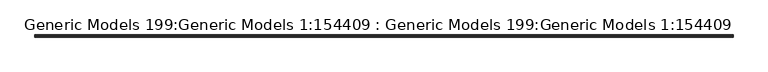
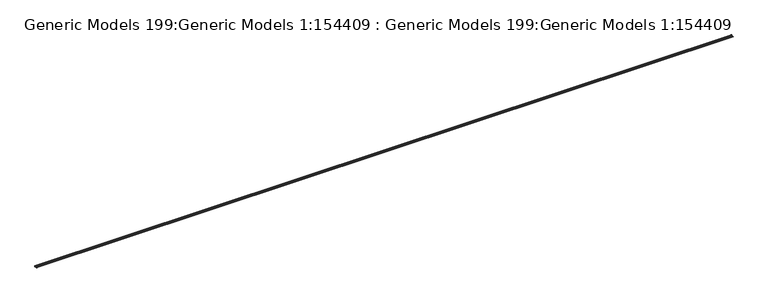
"""IFC4 building model written with IfcOpenShell, lengths in millimetres: proxy geometry, Generic Models 199:Generic Models 1:154409 : Generic Models 199:Generic Models 1:154409."""

from ifc_helpers import new_model, si_unit, frame, origin, place, context, project, spatial, polyline, outline, extrude, source, transform, mapped, element, save


def generic_models_199_generic_models_1_154409_generic_models_aefc242c(model_context):
    return source(origin(), model_context, "Body", "SweptSolid", [
        extrude(outline(polyline([(12159.4075942, 3046.095), (12179.0925942, 3046.095), (12179.0925942, 3048.3048), (12178.2337533, 3048.3048), (12178.2337533, 3068.6193787), (12179.5037533, 3068.6193787), (12179.5037533, 3049.5748), (12180.3625942, 3049.5748), (12180.3625942, 3044.825), (12158.1375942, 3044.825), (12158.1375942, 3056.255), (12145.4375942, 3056.255), (12145.4375942, 3044.825), (12121.7244102, 3044.825), (12121.7244102, 3046.095), (12144.1675942, 3046.095), (12144.1675942, 3057.525), (12159.4075942, 3057.525), (12159.4075942, 3046.095)])), frame((-10588.6040248, 0.0, 0.0), z_axis=(1.0, 0.0, 0.0), x_axis=(0.0, 1.0, 0.0)), (0.0, 0.0, 1.0), 19050.0),
    ])


if __name__ == "__main__":
    model = new_model("IFC4")
    model_context = context("Model", 3, world=origin())
    ifc_project = project(units=[si_unit("LENGTHUNIT", "METRE", prefix="MILLI")], contexts=[model_context])
    site = spatial("IfcSite", under=ifc_project)
    building = spatial("IfcBuilding", under=site)
    placement = place(None, origin())
    generic_models_199_generic_models_1_154409_generic_models_shape = generic_models_199_generic_models_1_154409_generic_models_aefc242c(model_context)
    element("IfcBuildingElementProxy", 1, Name="Generic Models 199:Generic Models 1:154409 : Generic Models 199:Generic Models 1:154409", ObjectType="Generic Models 199:Generic Models 1:154409 : Generic Models 199:Generic Models 1:154409", at=placement, inside=building, context=model_context, shape_type="MappedRepresentation", body=[
        mapped(generic_models_199_generic_models_1_154409_generic_models_shape, transform((0.0, 0.0, 0.0), x_axis=(1.0, 0.0, 0.0), y_axis=(0.0, 1.0, 0.0), z_axis=(0.0, 0.0, 1.0))),
    ])
    save(model, "model.ifc")

# Revit data of these elements
# Type "Generic Models 199:Generic Models 1:154409 : Generic Models 199:Generic Models 1:154409"
#   NameOverride = "Generic Models 199:Generic Models 1:154409"
#   ObjectTypeOverride = "Generic Models 199:Generic Models 1"
#   Reference = "Generic Models 1"
#   Category = "Generic Models"
#   Tag = "154409"
# Element 1 (IfcBuildingElementProxy, "Generic Models 199:Generic Models 1:154409 : Generic Models 199:Generic Models 1:154409")
#   Materials on its faces: "_16 GA. COPPER SOFFIT DRIP SCREED 1359"
# Materials
#   "_16 GA. COPPER SOFFIT DRIP SCREED 1359": class "Unassigned", colour RGB 253 192 103, transparency 0
